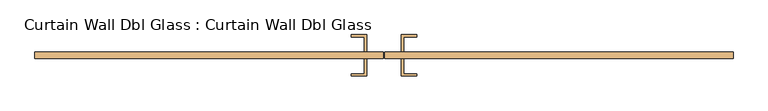
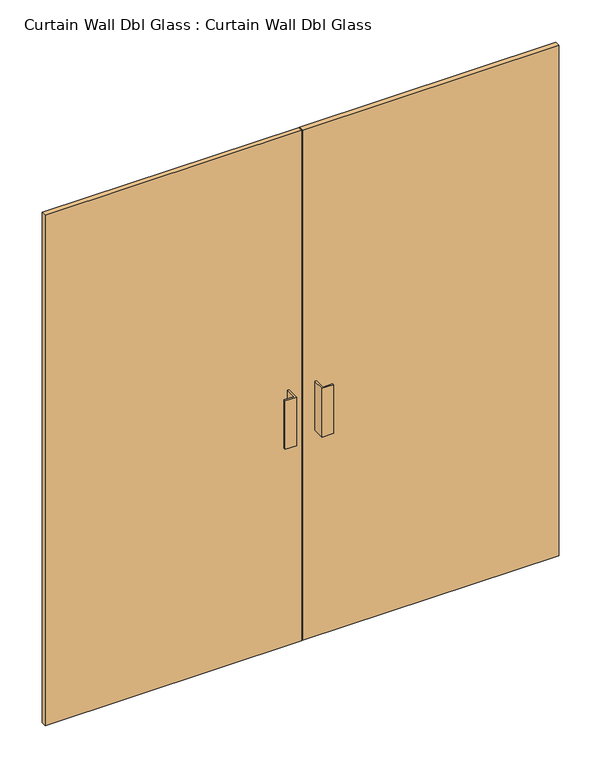
"""IFC4 building model written with IfcOpenShell, lengths in millimetres: door geometry, Curtain Wall Dbl Glass : Curtain Wall Dbl Glass."""

from ifc_helpers import new_model, si_unit, frame, origin, origin_with_axes, place, context, project, spatial, polyline, outline, extrude, source, transform, mapped, element, save


def curtain_wall_dbl_glass_curtain_wall_dbl_glass_d7d74fe3(model_context):
    return source(origin(), model_context, "Body", "SweptSolid", [
        extrude(outline(polyline([(-1.5875, 31.75), (-1016.0, 31.75), (-1016.0, 50.8), (-1.5875, 50.8), (-1.5875, 31.75)])), origin_with_axes(), (0.0, 0.0, 1.0), 2133.6),
        extrude(outline(polyline([(1016.0, 31.75), (1.5875, 31.75), (1.5875, 50.8), (1016.0, 50.8), (1016.0, 31.75)])), origin_with_axes(), (0.0, 0.0, 1.0), 2133.6),
        extrude(outline(polyline([(-50.8, 101.6), (-50.8, 50.8), (-57.15, 50.8), (-57.15, 95.25), (-95.25, 95.25), (-95.25, 101.6), (-50.8, 101.6)])), frame((0.0, 0.0, 863.6), z_axis=(0.0, 0.0, 1.0), x_axis=(1.0, 0.0, 0.0)), (0.0, 0.0, 1.0), 203.2),
        extrude(outline(polyline([(50.8, 101.6), (95.25, 101.6), (95.25, 95.25), (57.15, 95.25), (57.15, 50.8), (50.8, 50.8), (50.8, 101.6)])), frame((0.0, 0.0, 863.6), z_axis=(0.0, 0.0, 1.0), x_axis=(1.0, 0.0, 0.0)), (0.0, 0.0, 1.0), 203.2),
        extrude(outline(polyline([(-50.8, -19.05), (-95.25, -19.05), (-95.25, -12.7), (-57.15, -12.7), (-57.15, 31.75), (-50.8, 31.75), (-50.8, -19.05)])), frame((0.0, 0.0, 863.6), z_axis=(0.0, 0.0, 1.0), x_axis=(1.0, 0.0, 0.0)), (0.0, 0.0, 1.0), 203.2),
        extrude(outline(polyline([(50.8, -19.05), (50.8, 31.75), (57.15, 31.75), (57.15, -12.7), (95.25, -12.7), (95.25, -19.05), (50.8, -19.05)])), frame((0.0, 0.0, 863.6), z_axis=(0.0, 0.0, 1.0), x_axis=(1.0, 0.0, 0.0)), (0.0, 0.0, 1.0), 203.2),
    ])


if __name__ == "__main__":
    model = new_model("IFC4")
    model_context = context("Model", 3, world=origin())
    ifc_project = project(units=[si_unit("LENGTHUNIT", "METRE", prefix="MILLI")], contexts=[model_context])
    site = spatial("IfcSite", under=ifc_project)
    building = spatial("IfcBuilding", under=site)
    placement = place(None, origin())
    curtain_wall_dbl_glass_curtain_wall_dbl_glass_shape = curtain_wall_dbl_glass_curtain_wall_dbl_glass_d7d74fe3(model_context)
    element("IfcDoor", 1, ObjectType="Curtain Wall Dbl Glass : Curtain Wall Dbl Glass", at=placement, inside=building, context=model_context, shape_type="MappedRepresentation", body=[
        mapped(curtain_wall_dbl_glass_curtain_wall_dbl_glass_shape, transform((0.0, 0.0, 0.0), x_axis=(1.0, 0.0, 0.0), y_axis=(0.0, 1.0, 0.0), z_axis=(0.0, 0.0, 1.0))),
    ])
    save(model, "model.ifc")

# Revit data of these elements
# Type "Curtain Wall Dbl Glass : Curtain Wall Dbl Glass"
#   Offset = 0' - 2"
#   Function = 1
#   Handle Material = Metal - Aluminum
#   Glazing Material = Glass
# Element 1 (IfcDoor, "Curtain Wall Dbl Glass : Curtain Wall Dbl Glass")
#   Materials on its faces: "Metal - Aluminum", "Glass"
# Materials
#   "Metal - Aluminum": class "Metal", colour RGB 140 140 140, transparency 0
#   "Glass": class "Glass", colour RGB 0 128 192, transparency 0.75
